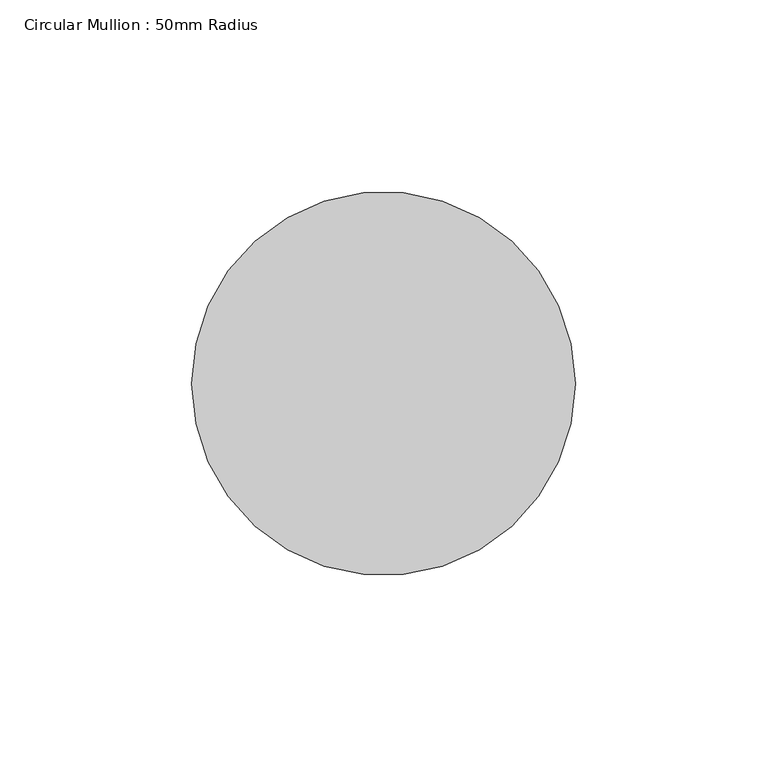
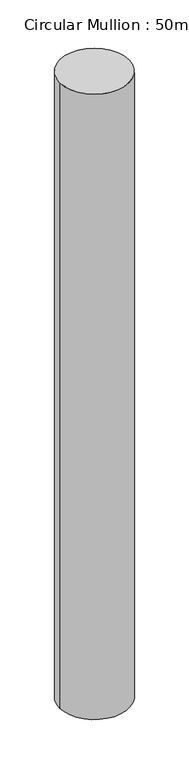
"""IFC4 building model written with IfcOpenShell, lengths in millimetres: member geometry, Circular Mullion : 50mm Radius."""

import ifcopenshell
import ifcopenshell.guid

model = None  # the IFC model being written
_history = None  # IfcOwnerHistory: only IFC2X3 demands one
_inside = {}  # id of a spatial element -> (the spatial element, [elements in it])
_under = {}  # id of a project, library or spatial element -> (it, [spatial elements below it])
_declared = {}  # id of a project -> (the project, [libraries it declares])
_typed = {}  # id of a type object -> (the type object, [elements of that type])
_made_of = {}  # id of a material, layer set ... -> (it, [elements and type objects made of it])


def new_model(schema):
    """Start an empty IFC model of exactly this schema.

    Asked for "IFC4X3", IfcOpenShell would pick the latest addendum, in which some entities
    have other attributes; the version numbers below select the first issue.
    IFC2X3 requires an IfcOwnerHistory on every rooted entity: one is made here for all.
    """
    global model, _history
    if schema == "IFC4X3":
        model = ifcopenshell.file(schema_version=(4, 3, 0, 0))
    else:
        model = ifcopenshell.file(schema=schema)
    _inside.clear()
    _under.clear()
    _declared.clear()
    _typed.clear()
    _made_of.clear()
    _history = None
    if model.schema == "IFC2X3":
        org = make("IfcOrganization", Name="unknown")
        user = make(
            "IfcPersonAndOrganization",
            ThePerson=make("IfcPerson", FamilyName="unknown"),
            TheOrganization=org,
        )
        app = make(
            "IfcApplication",
            ApplicationDeveloper=org,
            Version="unknown",
            ApplicationFullName="unknown",
            ApplicationIdentifier="unknown",
        )
        _history = make(
            "IfcOwnerHistory",
            OwningUser=user,
            OwningApplication=app,
            ChangeAction="ADDED",
            CreationDate=0,
        )
    return model


def make(cls, **values):
    """One entity of the class cls with the attributes given. An attribute that is None is left unset."""
    return model.create_entity(
        cls, **{name: value for name, value in values.items() if value is not None}
    )


def rooted(cls, **values):
    """An entity with a GlobalId (a new one), such as an element, a storey or a relation."""
    return make(cls, GlobalId=ifcopenshell.guid.new(), OwnerHistory=_history, **values)


def si_unit(unit_type, name, prefix=None):
    """IfcSIUnit, for example si_unit("LENGTHUNIT", "METRE", prefix="MILLI")."""
    return make("IfcSIUnit", UnitType=unit_type, Prefix=prefix, Name=name)


def assignment(units):
    """IfcUnitAssignment: the units of a project."""
    return None if units is None else make("IfcUnitAssignment", Units=units)


def point(xyz):
    """IfcCartesianPoint."""
    return None if xyz is None else make("IfcCartesianPoint", Coordinates=xyz)


def direction(xyz):
    """IfcDirection."""
    return None if xyz is None else make("IfcDirection", DirectionRatios=xyz)


def frame(location, z_axis=None, x_axis=None):
    """IfcAxis2Placement3D, a coordinate frame: its origin and axes. An axis left out is left unset."""
    return make(
        "IfcAxis2Placement3D",
        Location=point(location),
        Axis=direction(z_axis),
        RefDirection=direction(x_axis),
    )


def frame_2d(location, x_axis=None):
    """IfcAxis2Placement2D, a coordinate frame in the plane: its origin and x axis."""
    return make(
        "IfcAxis2Placement2D", Location=point(location), RefDirection=direction(x_axis)
    )


def origin():
    """The frame at (0, 0, 0) with its axes left unset."""
    return frame((0.0, 0.0, 0.0))


def origin_2d():
    """The frame at (0, 0) in the plane with its x axis left unset."""
    return frame_2d((0.0, 0.0))


def place(relative_to, where):
    """IfcLocalPlacement: puts the frame where relative to a parent placement (None: the world)."""
    return make(
        "IfcLocalPlacement", PlacementRelTo=relative_to, RelativePlacement=where
    )


def context(
    kind, dimensions, precision=None, world=None, true_north=None, identifier=None
):
    """IfcGeometricRepresentationContext, for example the 3D "Model" context."""
    return make(
        "IfcGeometricRepresentationContext",
        ContextIdentifier=identifier,
        ContextType=kind,
        CoordinateSpaceDimension=dimensions,
        Precision=precision,
        WorldCoordinateSystem=world,
        TrueNorth=true_north,
    )


def project(units=None, contexts=None):
    """IfcProject with its units and contexts."""
    return rooted(
        "IfcProject",
        Name="project",
        RepresentationContexts=contexts,
        UnitsInContext=assignment(units),
    )


def spatial(cls, under=None, at=None, **own):
    """A site, building, storey or space (cls), placed at a placement, below another one or the project."""
    s = rooted(cls, ObjectPlacement=at, **own)
    if under is not None:
        _under.setdefault(under.id(), (under, []))[1].append(s)
    return s


def circle_curve(where, radius):
    """IfcCircle in the frame where."""
    return make("IfcCircle", Position=where, Radius=radius)


def trimmed(basis, trim1, trim2, sense, master):
    """IfcTrimmedCurve: the piece of a basis curve between two trims."""
    return make(
        "IfcTrimmedCurve",
        BasisCurve=basis,
        Trim1=trim1,
        Trim2=trim2,
        SenseAgreement=sense,
        MasterRepresentation=master,
    )


def segment(curve, same_sense, transition):
    """IfcCompositeCurveSegment."""
    return make(
        "IfcCompositeCurveSegment",
        Transition=transition,
        SameSense=same_sense,
        ParentCurve=curve,
    )


def composite_curve(segments, self_intersect=None):
    """IfcCompositeCurve: segments joined end to end."""
    return make("IfcCompositeCurve", Segments=segments, SelfIntersect=self_intersect)


def outline(outer, holes=None, kind="AREA"):
    """IfcArbitraryClosedProfileDef: a profile drawn as a closed curve; with holes, ...WithVoids."""
    if holes is None:
        return make("IfcArbitraryClosedProfileDef", ProfileType=kind, OuterCurve=outer)
    return make(
        "IfcArbitraryProfileDefWithVoids",
        ProfileType=kind,
        OuterCurve=outer,
        InnerCurves=holes,
    )


def extrude(swept, where, along, depth):
    """IfcExtrudedAreaSolid: the profile swept, set in the frame where, extruded along a direction by depth."""
    return make(
        "IfcExtrudedAreaSolid",
        SweptArea=swept,
        Position=where,
        ExtrudedDirection=direction(along),
        Depth=depth,
    )


def shape(context_of_items, identifier, shape_type, items):
    """IfcShapeRepresentation: the items that make up one representation, for example the "Body"."""
    return make(
        "IfcShapeRepresentation",
        ContextOfItems=context_of_items,
        RepresentationIdentifier=identifier,
        RepresentationType=shape_type,
        Items=items,
    )


def source(mapping_origin, context_of_items, identifier, shape_type, items):
    """IfcRepresentationMap: a shape defined once, which mapped items show again and again."""
    return make(
        "IfcRepresentationMap",
        MappingOrigin=mapping_origin,
        MappedRepresentation=shape(context_of_items, identifier, shape_type, items),
    )


def transform(
    local_origin,
    x_axis=None,
    y_axis=None,
    z_axis=None,
    scale=None,
    scale2=None,
    scale3=None,
    uniform=True,
):
    """IfcCartesianTransformationOperator3D, or its non-uniform kind. x_axis, y_axis, z_axis: its Axis1, 2, 3."""
    if uniform:
        return make(
            "IfcCartesianTransformationOperator3D",
            Axis1=direction(x_axis),
            Axis2=direction(y_axis),
            LocalOrigin=point(local_origin),
            Scale=scale,
            Axis3=direction(z_axis),
        )
    return make(
        "IfcCartesianTransformationOperator3DnonUniform",
        Axis1=direction(x_axis),
        Axis2=direction(y_axis),
        LocalOrigin=point(local_origin),
        Scale=scale,
        Axis3=direction(z_axis),
        Scale2=scale2,
        Scale3=scale3,
    )


def mapped(mapping_source, mapping_target):
    """IfcMappedItem: shows the shape of a source again, moved by a transform."""
    return make(
        "IfcMappedItem", MappingSource=mapping_source, MappingTarget=mapping_target
    )


def made_of(thing, what):
    """Note that an element or type object is made of a material, layer set ...; save() writes the relation."""
    if what is not None:
        _made_of.setdefault(what.id(), (what, []))[1].append(thing)
    return thing


def element(
    cls,
    number,
    at=None,
    inside=None,
    cuts=None,
    type_object=None,
    material=None,
    context=None,
    identifier="Body",
    shape_type=None,
    held_by="IfcProductDefinitionShape",
    body=None,
    shapes=None,
    **own,
):
    """One element of the class cls, such as IfcWall. Its Tag is "e" and its number.

    at: its placement. inside: the storey or other place that contains it. cuts: it is an
    opening in that element (IfcRelVoidsElement). A single representation is given by context,
    identifier, shape_type and body (its items); several are given by shapes. held_by: the class
    of the entity that holds the representations. save() writes the other relations.
    """
    e = rooted(cls, Tag="e%d" % number, ObjectPlacement=at, **own)
    if body is not None:
        shapes = [shape(context, identifier, shape_type, body)]
    if shapes is not None:
        e.Representation = make(held_by, Representations=shapes)
    if inside is not None:
        _inside.setdefault(inside.id(), (inside, []))[1].append(e)
    if cuts is not None:
        rooted(
            "IfcRelVoidsElement", RelatingBuildingElement=cuts, RelatedOpeningElement=e
        )
    if type_object is not None:
        _typed.setdefault(type_object.id(), (type_object, []))[1].append(e)
    return made_of(e, material)


def aggregate(whole, parts):
    """IfcRelAggregates: a whole, such as a stair, and the parts it consists of."""
    return rooted("IfcRelAggregates", RelatingObject=whole, RelatedObjects=parts)


def save(model, path):
    """Write the relations noted so far, then the file.

    IfcRelAggregates (storeys below a building ...), IfcRelContainedInSpatialStructure (elements
    in a storey), IfcRelDefinesByType, IfcRelAssociatesMaterial and IfcRelDeclares: one each for
    every whole, place, type object, material and project.
    """
    for whole, parts in _under.values():
        aggregate(whole, parts)
    for where, things in _inside.values():
        rooted(
            "IfcRelContainedInSpatialStructure",
            RelatedElements=things,
            RelatingStructure=where,
        )
    for kind, things in _typed.values():
        rooted("IfcRelDefinesByType", RelatedObjects=things, RelatingType=kind)
    for what, things in _made_of.values():
        rooted("IfcRelAssociatesMaterial", RelatedObjects=things, RelatingMaterial=what)
    for by, libraries in _declared.values():
        rooted("IfcRelDeclares", RelatingContext=by, RelatedDefinitions=libraries)
    model.write(path)


def circular_mullion_50mm_radius_d3c402de(model_context):
    return source(origin(), model_context, "Body", "SweptSolid", [
        extrude(outline(composite_curve([segment(trimmed(circle_curve(origin_2d(), 50.0), [point((50.0, 0.0))], [point((-50.0, 0.0))], False, "CARTESIAN"), True, "CONTINUOUS"), segment(trimmed(circle_curve(origin_2d(), 50.0), [point((-50.0, 0.0))], [point((50.0, 0.0))], False, "CARTESIAN"), True, "CONTINUOUS")], self_intersect=False)), frame((0.0, 0.0, -954.5686159), z_axis=(0.0, 0.0, 1.0), x_axis=(1.0, 0.0, 0.0)), (0.0, 0.0, 1.0), 954.5686159),
    ])


if __name__ == "__main__":
    model = new_model("IFC4")
    model_context = context("Model", 3, world=origin())
    ifc_project = project(units=[si_unit("LENGTHUNIT", "METRE", prefix="MILLI")], contexts=[model_context])
    site = spatial("IfcSite", under=ifc_project)
    building = spatial("IfcBuilding", under=site)
    placement = place(None, origin())
    circular_mullion_50mm_radius_shape = circular_mullion_50mm_radius_d3c402de(model_context)
    element("IfcMember", 1, ObjectType="Circular Mullion : 50mm Radius", at=placement, inside=building, context=model_context, shape_type="MappedRepresentation", body=[
        mapped(circular_mullion_50mm_radius_shape, transform((0.0, 0.0, 0.0), x_axis=(1.0, 0.0, 0.0), y_axis=(0.0, 1.0, 0.0), z_axis=(0.0, 0.0, 1.0))),
    ])
    save(model, "model.ifc")

# Revit data of these elements
# Type "Circular Mullion : 50mm Radius"
#   built-in parameter 1007350 = 0.164042 (stored number, unit not read)
# Element 1 (IfcMember, "Circular Mullion : 50mm Radius")
#   Materials on its faces: "Aluminium"
# Materials
#   "Aluminium": class "Metal", colour RGB 247 247 247, transparency 0, Description = "Aluminium 6061", Cost = 0
